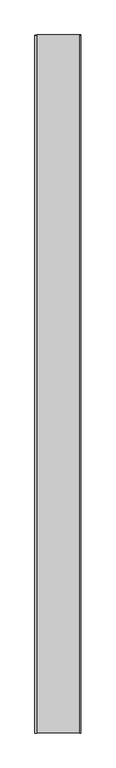
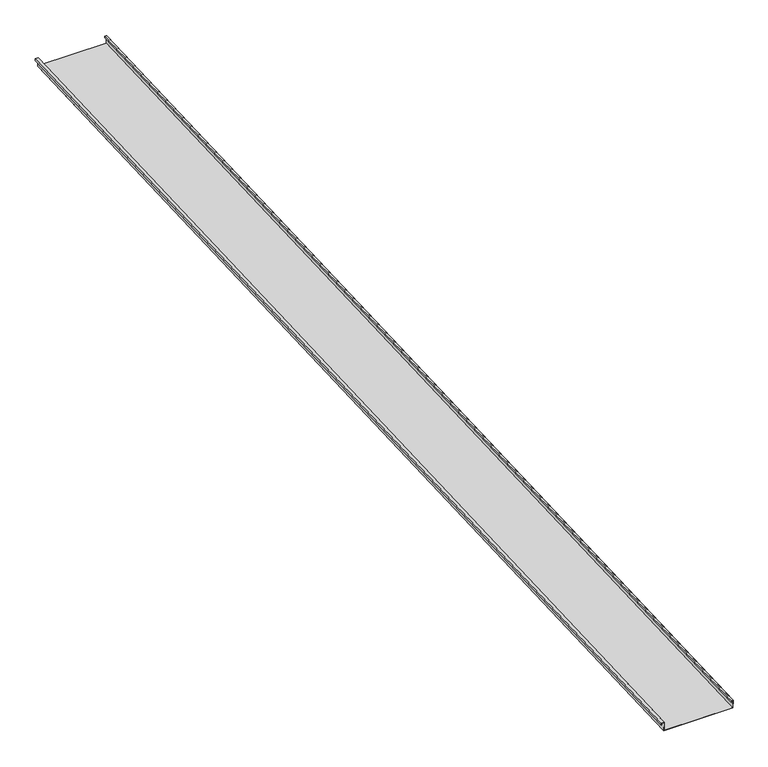
"""IFC4 building model written with IfcOpenShell, lengths in millimetres: proxy geometry, Generic Models 2:Generic Models 2:310765:Generic Models 2:310765 : Generic Models 2:Generic Models 2:310765:101 : Generic Models 2:Generic Models 2:310765:Generic Models 2:310765 : Generic Models 2:Generic Models 2:310765:300385."""

from ifc_helpers import new_model, si_unit, frame, origin, place, context, project, spatial, polyline, outline, extrude, source, transform, mapped, element, save


def generic_models_c5d6812a(model_context):
    return source(origin(), model_context, "Body", "SweptSolid", [
        extrude(outline(polyline([(1.5875, 0.0), (1.5875, 50.8), (407.9875, 50.8), (407.9875, 1.5875), (396.875, 1.5875), (396.875, 11.1125), (398.4625, 11.1125), (398.4625, 3.175), (406.4, 3.175), (406.4, 49.2125), (3.175, 49.2125), (3.175, -1.5874999), (-14.2875, -1.5874999), (-14.2875, 9.525), (-12.7, 9.525), (-12.7, 0.0), (1.5875, 0.0)])), frame((612736.4929739, -581354.4345603, 3902.6697972), z_axis=(0.0, 0.9991330730923568, 0.041630544712067834), x_axis=(1.0, 0.0, 0.0)), (0.0, 0.0, 1.0), 6400.8),
    ])


if __name__ == "__main__":
    model = new_model("IFC4")
    model_context = context("Model", 3, world=origin())
    ifc_project = project(units=[si_unit("LENGTHUNIT", "METRE", prefix="MILLI")], contexts=[model_context])
    site = spatial("IfcSite", under=ifc_project)
    building = spatial("IfcBuilding", under=site)
    placement = place(None, origin())
    generic_models_shape = generic_models_c5d6812a(model_context)
    element("IfcBuildingElementProxy", 1, Name="Generic Models 2:Generic Models 2:310765:Generic Models 2:310765 : Generic Models 2:Generic Models 2:310765:101 : Generic Models 2:Generic Models 2:310765:Generic Models 2:310765 : Generic Models 2:Generic Models 2:310765:300385", ObjectType="Generic Models 2:Generic Models 2:310765:Generic Models 2:310765 : Generic Models 2:Generic Models 2:310765:101 : Generic Models 2:Generic Models 2:310765:Generic Models 2:310765 : Generic Models 2:Generic Models 2:310765:300385", at=placement, inside=building, context=model_context, shape_type="MappedRepresentation", body=[
        mapped(generic_models_shape, transform((0.0, 0.0, 0.0), x_axis=(1.0, 0.0, 0.0), y_axis=(0.0, 1.0, 0.0), z_axis=(0.0, 0.0, 1.0))),
    ])
    save(model, "model.ifc")

# Revit data of these elements
# Type "Generic Models 2:Generic Models 2:310765:Generic Models 2:310765 : Generic Models 2:Generic Models 2:310765:101 : Generic Models 2:Generic Models 2:310765:Generic Models 2:310765 : Generic Models 2:Generic Models 2:310765:300385"
#   NameOverride = "Generic Models 2:Generic Models 2:310765:Generic Models 2:310765 : Generic Models 2:Generic Models 2:310765:300385"
#   ObjectTypeOverride = "Generic Models 2:310765 : Generic Models 2:Generic Models 2:310765"
#   Reference = "Generic Models 2"
#   Tag = "300385"
# Element 1 (IfcBuildingElementProxy, "Generic Models 2:Generic Models 2:310765:Generic Models 2:310765 : Generic Models 2:Generic Models 2:310765:101 : Generic Models 2:Generic Models 2:310765:Generic Models 2:310765 : Generic Models 2:Generic Models 2:310765:300385")
#   Materials on its faces: "THERMAL BROKEN ALUMINUM STOREFRONT FOR POLYCARBONATE"
# Materials
#   "THERMAL BROKEN ALUMINUM STOREFRONT FOR POLYCARBONATE": class "Unassigned", colour RGB 244 244 244, transparency 0, Keynote = "M07611300.01", Cost = 0
